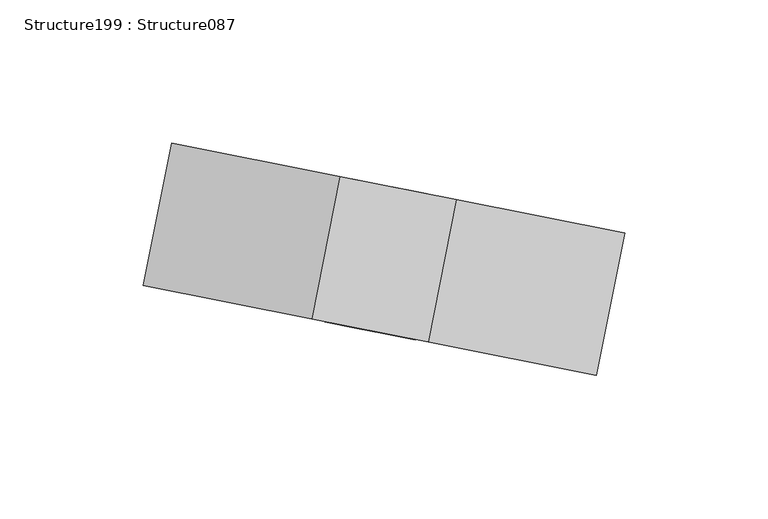
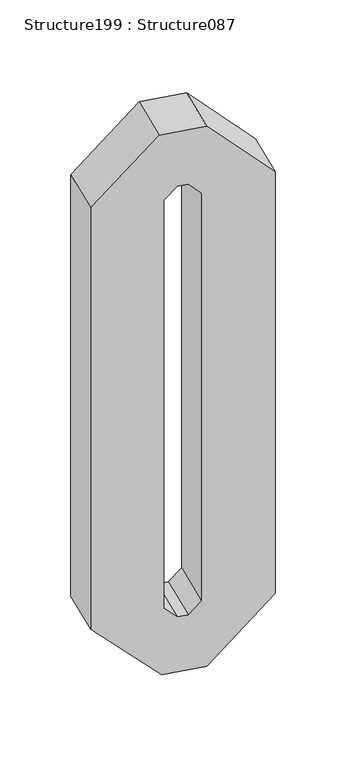
"""IFC4 building model written with IfcOpenShell, lengths in millimetres: proxy geometry, Structure199 : Structure087."""

from ifc_helpers import new_model, si_unit, frame, origin, place, context, project, spatial, polyline, outline, extrude, source, transform, mapped, element, save


def structure199_structure087_4c6ea098(model_context):
    return source(origin(), model_context, "Body", "SweptSolid", [
        extrude(outline(polyline([(425.6202752, 0.0), (485.5454951, -59.9250697), (485.5454951, -101.4135448), (425.6204255, -161.3386144), (-0.0006857, -161.3379027), (-59.8837361, -99.1882103), (-59.9250696, -59.9250697), (0.0, 0.0), (425.6202752, 0.0)]), holes=[polyline([(-4.610305, -85.2790785), (6.9144584, -96.8039514), (418.7015877, -96.8039514), (430.2261049, -85.2794343), (430.2261049, -76.0616708), (418.7015877, -64.5371537), (6.9145779, -64.5371537), (-4.6099492, -76.0616708), (-4.610305, -85.2790785)])]), frame((-1639.5402808, 234793.8588682, 652.0550604), z_axis=(0.19466222296394123, 0.9808703374813295, 0.0), x_axis=(0.0, 0.0, 1.0)), (0.0, 0.0, 1.0), 50.8),
    ])


if __name__ == "__main__":
    model = new_model("IFC4")
    model_context = context("Model", 3, world=origin())
    ifc_project = project(units=[si_unit("LENGTHUNIT", "METRE", prefix="MILLI")], contexts=[model_context])
    site = spatial("IfcSite", under=ifc_project)
    building = spatial("IfcBuilding", under=site)
    placement = place(None, origin())
    structure199_structure087_shape = structure199_structure087_4c6ea098(model_context)
    element("IfcBuildingElementProxy", 1, Name="Structure199 : Structure087", ObjectType="Structure199 : Structure087", at=placement, inside=building, context=model_context, shape_type="MappedRepresentation", body=[
        mapped(structure199_structure087_shape, transform((0.0, 0.0, 0.0), x_axis=(1.0, 0.0, 0.0), y_axis=(0.0, 1.0, 0.0), z_axis=(0.0, 0.0, 1.0))),
    ])
    save(model, "model.ifc")

# Revit data of these elements
# Type "Structure199 : Structure087"
#   NameOverride = "Structure087"
# Element 1 (IfcBuildingElementProxy, "Structure199 : Structure087")
#   Materials on its faces: "BRUSHED ALUMINUM LETTERING"
# Materials
#   "BRUSHED ALUMINUM LETTERING": class "Unassigned", colour RGB 169 181 186, transparency 0, Cost = 0
